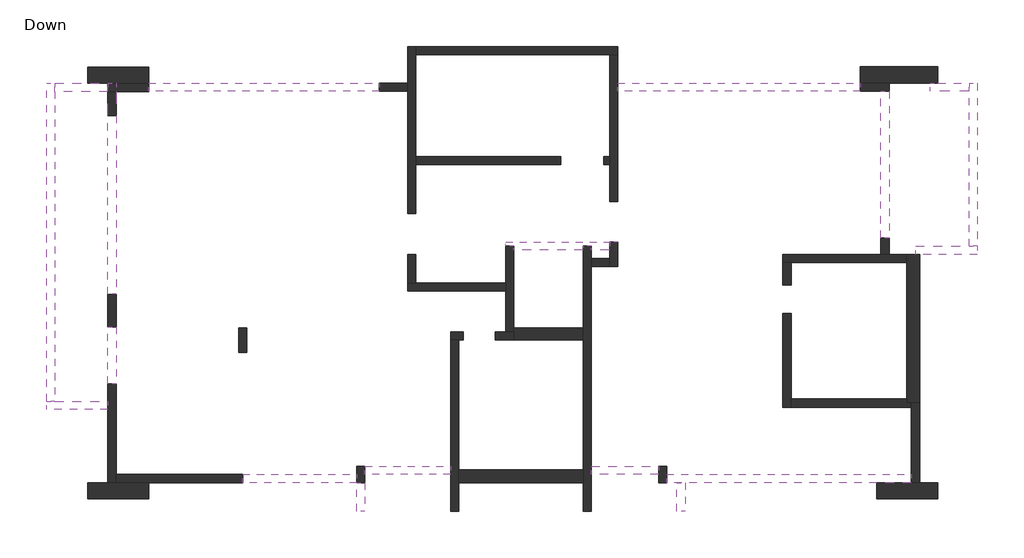
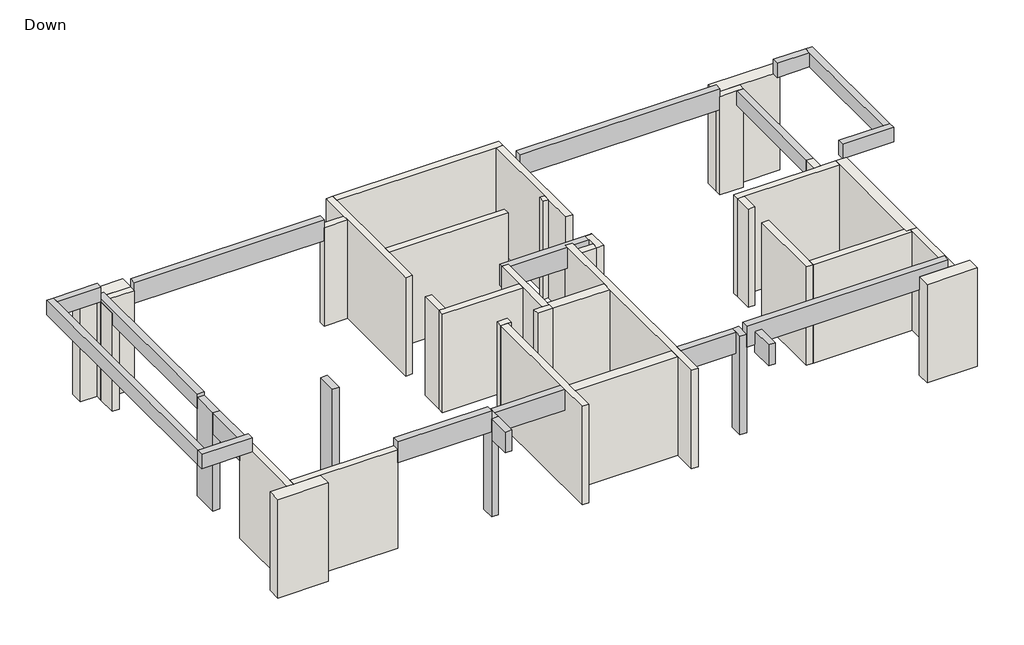
# One storey: 33 walls, 18 beams, 4 columns.
"""IFC4 building model written with IfcOpenShell, lengths in millimetres."""

from ifc_helpers import new_model, si_unit, frame, origin, origin_with_axes, place, context, project, spatial, polyline, outline, extrude, faceted_brep, element, save

model = new_model("IFC4")

# Units and contexts
model_context = context("Model", 3, world=origin())
ifc_project = project(units=[si_unit("LENGTHUNIT", "METRE", prefix="MILLI")], contexts=[model_context])

# Site, building, storey
site = spatial("IfcSite", under=ifc_project)
building = spatial("IfcBuilding", under=site)
storey = spatial("IfcBuildingStorey", under=building, Name="Down", Elevation=0.0)

# Beams
placement = place(None, origin())
element("IfcBeam", 1, ObjectType="Concrete Rectengular Beam : 20/45", at=placement, inside=storey, context=model_context, shape_type="Brep", body=[
    faceted_brep([(-51622.338535, 14321.5649818, 3200.0), (-51822.338535, 14321.5649818, 3200.0), (-51822.338535, 14321.5649818, 2750.0), (-51622.338535, 14321.5649818, 2750.0), (-51622.338535, 19497.0389138, 3200.0), (-51822.338535, 19497.0389138, 3200.0), (-51822.338535, 19497.0389138, 3100.0), (-51822.338535, 19297.0389138, 3100.0), (-51822.338535, 18701.2717181, 3100.0), (-51822.338535, 18701.2717181, 2750.0), (-51622.338535, 18701.2717181, 2750.0), (-51622.338535, 18701.2717181, 3100.0), (-51622.338535, 19297.0389138, 3100.0), (-51622.338535, 19497.0389138, 3100.0)], [[[0, 1, 2, 3]], [[1, 0, 4, 5]], [[2, 1, 5, 6, 7, 8, 9]], [[3, 2, 9, 10]], [[0, 3, 10, 11, 12, 13, 4]], [[5, 4, 13, 6]], [[6, 13, 12, 11, 8, 7]], [[8, 11, 10, 9]]]),
])
element("IfcBeam", 2, ObjectType="Concrete Rectengular Beam : 20/45", at=placement, inside=storey, context=model_context, shape_type="Brep", body=[
    faceted_brep([(-32674.1903869, 19301.2717181, 3100.0), (-32874.1903869, 19301.2717181, 3100.0), (-32874.1903869, 15700.213517, 3100.0), (-32674.1903869, 15700.213517, 3100.0), (-32674.1903869, 19301.2717181, 2650.0), (-32674.1903869, 19301.2717181, 2850.0), (-32674.1903869, 15700.213517, 2650.0), (-32874.1903869, 19301.2717181, 2650.0), (-32874.1903869, 15700.213517, 2650.0), (-32874.1903869, 19301.2717181, 2850.0), (-32874.1903869, 15700.213517, 2850.0)], [[[0, 1, 2, 3]], [[4, 5, 0, 3, 6]], [[7, 4, 6, 8]], [[2, 1, 9, 7, 8, 10]], [[1, 0, 5, 4, 7, 9]], [[3, 2, 10, 8, 6]]]),
])
element("IfcBeam", 3, ObjectType="Concrete Rectengular Beam : 20/45", at=placement, inside=storey, context=model_context, shape_type="Brep", body=[
    faceted_brep([(-32023.9258366, 15500.213517, 3550.0), (-32023.9258366, 15500.213517, 3100.0), (-32023.9258366, 15300.213517, 3100.0), (-32023.9258366, 15300.213517, 3550.0), (-30505.8186523, 15300.213517, 3550.0), (-30505.8186523, 15500.213517, 3550.0), (-30705.8186523, 15500.213517, 3550.0), (-30505.8186523, 15300.213517, 3100.0), (-30705.8186523, 15500.213517, 3100.0), (-30505.8186523, 15500.213517, 3100.0)], [[[0, 1, 2, 3]], [[0, 3, 4, 5, 6]], [[3, 2, 7, 4]], [[2, 1, 8, 9, 7]], [[1, 0, 6, 5, 9, 8]], [[5, 4, 7, 9]]]),
])
element("IfcBeam", 4, ObjectType="Concrete Rectengular Beam : 20/45", at=placement, inside=storey, context=model_context, shape_type="Brep", body=[
    faceted_brep([(-30505.8186523, 19501.2717181, 3550.0), (-30705.8186523, 19501.2717181, 3550.0), (-30705.8186523, 19301.2717181, 3550.0), (-30705.8186523, 15500.213517, 3550.0), (-30505.8186523, 15500.213517, 3550.0), (-30505.8186523, 19501.2717181, 3100.0), (-30505.8186523, 15500.213517, 3100.0), (-30705.8186523, 19501.2717181, 3100.0), (-30705.8186523, 15500.213517, 3100.0), (-30705.8186523, 19301.2717181, 3100.0)], [[[0, 1, 2, 3, 4]], [[5, 0, 4, 6]], [[7, 5, 6, 8, 9]], [[1, 7, 9, 8, 3, 2]], [[1, 0, 5, 7]], [[4, 3, 8, 6]]]),
])
element("IfcBeam", 5, ObjectType="Concrete Rectengular Beam : 20/45", at=placement, inside=storey, context=model_context, shape_type="Brep", body=[
    faceted_brep([(-31665.8186523, 19301.2717181, 3550.0), (-31665.8186523, 19501.2717181, 3550.0), (-31665.8186523, 19501.2717181, 3100.0), (-31665.8186523, 19301.2717181, 3100.0), (-30705.8186523, 19301.2717181, 3550.0), (-30705.8186523, 19501.2717181, 3550.0), (-30705.8186523, 19501.2717181, 3100.0), (-31473.1321858, 19501.2717181, 3100.0), (-30705.8186523, 19301.2717181, 3100.0)], [[[0, 1, 2, 3]], [[1, 0, 4, 5]], [[2, 1, 5, 6, 7]], [[3, 2, 7, 6, 8]], [[0, 3, 8, 4]], [[5, 4, 8, 6]]]),
])
element("IfcBeam", 6, ObjectType="Concrete Rectengular Beam : 20/45", at=placement, inside=storey, context=model_context, shape_type="Brep", body=[
    faceted_brep([(-51822.338535, 11493.9394503, 3550.0), (-51822.338535, 11493.9394503, 3100.0), (-51822.338535, 11693.9394503, 3100.0), (-51822.338535, 11693.9394503, 3550.0), (-53128.1898421, 11693.9394503, 3550.0), (-53328.1898421, 11693.9394503, 3550.0), (-53328.1898421, 11493.9394503, 3550.0), (-53128.1898421, 11693.9394503, 3100.0), (-53328.1898421, 11693.9394503, 3100.0), (-53328.1898421, 11493.9394503, 3100.0)], [[[0, 1, 2, 3]], [[0, 3, 4, 5, 6]], [[3, 2, 7, 8, 5, 4]], [[2, 1, 9, 8, 7]], [[1, 0, 6, 9]], [[6, 5, 8, 9]]]),
])
element("IfcBeam", 7, ObjectType="Concrete Rectengular Beam : 20/45", at=placement, inside=storey, context=model_context, shape_type="Brep", body=[
    faceted_brep([(-53128.1898421, 19497.0389138, 3550.0), (-53328.1898421, 19497.0389138, 3550.0), (-53328.1898421, 11693.9394503, 3550.0), (-53128.1898421, 11693.9394503, 3550.0), (-53128.1898421, 19297.0389138, 3550.0), (-53128.1898421, 19497.0389138, 3100.0), (-53128.1898421, 11693.9394503, 3100.0), (-53128.1898421, 19297.0389138, 3100.0), (-53328.1898421, 19497.0389138, 3100.0), (-53328.1898421, 11693.9394503, 3100.0)], [[[0, 1, 2, 3, 4]], [[5, 0, 4, 3, 6, 7]], [[8, 5, 7, 6, 9]], [[1, 8, 9, 2]], [[3, 2, 9, 6]], [[1, 0, 5, 8]]]),
])
element("IfcBeam", 8, ObjectType="Concrete Rectengular Beam : 20/45", at=placement, inside=storey, context=model_context, shape_type="Brep", body=[
    faceted_brep([(-51822.338535, 19497.0389138, 3550.0), (-51822.338535, 19297.0389138, 3550.0), (-51822.338535, 19297.0389138, 3100.0), (-51822.338535, 19497.0389138, 3100.0), (-51822.338535, 19497.0389138, 3200.0), (-53128.1898421, 19497.0389138, 3550.0), (-53128.1898421, 19297.0389138, 3550.0), (-53128.1898421, 19297.0389138, 3100.0), (-53128.1898421, 19497.0389138, 3100.0)], [[[0, 1, 2, 3, 4]], [[1, 0, 5, 6]], [[2, 1, 6, 7]], [[3, 2, 7, 8]], [[0, 4, 3, 8, 5]], [[6, 5, 8, 7]]]),
])
element("IfcBeam", 9, ObjectType="Concrete Rectengular Beam : 20/66", at=placement, inside=storey, context=model_context, shape_type="SweptSolid", body=[
    extrude(outline(polyline([(-51822.338535, 13521.5649818), (-51622.338535, 13521.5649818), (-51622.338535, 12125.6103424), (-51822.338535, 12125.6103424), (-51822.338535, 13521.5649818)])), frame((0.0, 0.0, 2440.0), z_axis=(0.0, 0.0, 1.0), x_axis=(1.0, 0.0, 0.0)), (0.0, 0.0, 1.0), 660.0),
])
element("IfcBeam", 10, ObjectType="Concrete Rectengular Beam : 20/66", at=placement, inside=storey, context=model_context, shape_type="Brep", body=[
    faceted_brep([(-45722.0604135, 9899.1553159, 3350.0), (-45722.0604135, 9699.1553159, 3350.0), (-45722.0604135, 9699.1553159, 3100.0), (-45722.0604135, 9699.1553159, 2690.0), (-45722.0604135, 9899.1553159, 2690.0), (-45722.0604135, 9899.1553159, 2850.0), (-45722.0604135, 9899.1553159, 3100.0), (-48520.2494744, 9899.1553159, 3350.0), (-48520.2494744, 9899.1553159, 2690.0), (-48520.2494744, 9699.1553159, 2690.0), (-48520.2494744, 9699.1553159, 3350.0)], [[[0, 1, 2, 3, 4, 5, 6]], [[7, 8, 9, 10]], [[1, 0, 7, 10]], [[3, 2, 1, 10, 9]], [[4, 3, 9, 8]], [[0, 6, 5, 4, 8, 7]]]),
])
element("IfcBeam", 11, ObjectType="Concrete Rectengular Beam : 20/66", at=placement, inside=storey, context=model_context, shape_type="Brep", body=[
    faceted_brep([(-45522.0604135, 10099.1553159, 3100.0), (-45522.0604135, 9899.1553159, 3100.0), (-43423.3967361, 9899.1553159, 3100.0), (-43423.3967361, 10099.1553159, 3100.0), (-45522.0604135, 9899.1553159, 2950.0), (-45522.0604135, 9899.1553159, 2440.0), (-43423.3967361, 9899.1553159, 2440.0), (-43423.3967361, 9899.1553159, 2950.0), (-45522.0604135, 10099.1553159, 2440.0), (-43423.3967361, 10099.1553159, 2440.0), (-43423.3967361, 10099.1553159, 2850.0), (-45522.0604135, 10099.1553159, 2850.0)], [[[0, 1, 2, 3]], [[1, 4, 5, 6, 7, 2]], [[5, 8, 9, 6]], [[0, 3, 10, 9, 8, 11]], [[1, 0, 11, 8, 5, 4]], [[3, 2, 7, 6, 9, 10]]]),
])
element("IfcBeam", 12, ObjectType="Concrete Rectengular Beam : 20/66", at=placement, inside=storey, context=model_context, shape_type="Brep", body=[
    faceted_brep([(-38322.0604135, 9899.1553159, 3100.0), (-38322.0604135, 10099.1553159, 3100.0), (-39973.6612863, 10099.1553159, 3100.0), (-39973.6612863, 9899.1553159, 3100.0), (-38322.0604135, 10099.1553159, 2850.0), (-38322.0604135, 10099.1553159, 2440.0), (-39973.6612863, 10099.1553159, 2440.0), (-39973.6612863, 10099.1553159, 2850.0), (-38322.0604135, 9899.1553159, 2440.0), (-39973.6612863, 9899.1553159, 2440.0), (-38322.0604135, 9899.1553159, 2950.0), (-39973.6612863, 9899.1553159, 2950.0)], [[[0, 1, 2, 3]], [[2, 1, 4, 5, 6, 7]], [[5, 8, 9, 6]], [[8, 10, 0, 3, 11, 9]], [[1, 0, 10, 8, 5, 4]], [[3, 2, 7, 6, 9, 11]]]),
])
element("IfcBeam", 13, ObjectType="Concrete Rectengular Beam : 20/66", at=placement, inside=storey, context=model_context, shape_type="Brep", body=[
    faceted_brep([(-32123.9258366, 9899.1553159, 2690.0), (-32123.9258366, 9899.1553159, 2850.0), (-32123.9258366, 9899.1553159, 3100.0), (-32123.9258366, 9899.1553159, 3350.0), (-32123.9258366, 9699.1553159, 3350.0), (-32123.9258366, 9699.1553159, 3100.0), (-32123.9258366, 9700.213517, 3100.0), (-32123.9258366, 9700.213517, 2690.0), (-38123.9258366, 9899.1553159, 3350.0), (-38123.9258366, 9699.1553159, 3350.0), (-38122.0604135, 9899.1553159, 2690.0), (-38122.0604135, 9899.1553159, 2850.0), (-38122.0604135, 9899.1553159, 3100.0), (-38123.9258366, 9899.1553159, 3100.0), (-38122.0604135, 9699.1553159, 2690.0), (-32973.6612863, 9700.213517, 2690.0), (-32973.6612863, 9699.1553159, 2690.0), (-38123.9258366, 9699.1553159, 3100.0), (-38122.0604135, 9699.1553159, 3100.0), (-38122.0604135, 9699.1553159, 2950.0), (-32973.6612863, 9699.1553159, 3100.0), (-32973.6612863, 9700.213517, 3100.0)], [[[0, 1, 2, 3, 4, 5, 6, 7]], [[4, 3, 8, 9]], [[3, 2, 1, 0, 10, 11, 12, 13, 8]], [[14, 10, 0, 7, 15, 16]], [[4, 9, 17, 18, 19, 14, 16, 20, 5]], [[18, 12, 11, 10, 14, 19]], [[12, 18, 17, 13]], [[6, 21, 15, 7]], [[21, 20, 16, 15]], [[20, 21, 6, 5]], [[9, 8, 13, 17]]]),
])
element("IfcBeam", 14, ObjectType="Concrete Rectengular Beam : 20/66", at=placement, inside=storey, context=model_context, shape_type="Brep", body=[
    faceted_brep([(-39322.8676355, 19301.2717181, 3350.0), (-39322.8676355, 19501.2717181, 3350.0), (-39322.8676355, 19501.2717181, 2690.0), (-39322.8676355, 19301.2717181, 2690.0), (-39322.8676355, 19301.2717181, 2850.0), (-39322.8676355, 19301.2717181, 3100.0), (-33373.6612863, 19301.2717181, 3350.0), (-33373.6612863, 19301.2717181, 3100.0), (-33373.6612863, 19301.2717181, 2690.0), (-33373.6612863, 19501.2717181, 2690.0), (-33373.6612863, 19501.2717181, 3100.0), (-33373.6612863, 19501.2717181, 3350.0)], [[[0, 1, 2, 3, 4, 5]], [[6, 7, 8, 9, 10, 11]], [[1, 0, 6, 11]], [[2, 1, 11, 10, 9]], [[3, 2, 9, 8]], [[0, 5, 4, 3, 8, 7, 6]]]),
])
element("IfcBeam", 15, ObjectType="Concrete Rectengular Beam : 20/66", at=placement, inside=storey, context=model_context, shape_type="Brep", body=[
    faceted_brep([(-39322.8676355, 15601.2717181, 3100.0), (-42072.0739847, 15601.2717181, 3100.0), (-42072.0739847, 15501.2717181, 3100.0), (-41872.0739847, 15501.2717181, 3100.0), (-41872.0739847, 15401.2717181, 3100.0), (-40173.6612863, 15401.2717181, 3100.0), (-40173.6612863, 15501.2717181, 3100.0), (-39973.6612863, 15501.2717181, 3100.0), (-39973.6612863, 15401.2717181, 3100.0), (-39522.8676355, 15401.2717181, 3100.0), (-39522.8676355, 15600.7426175, 3100.0), (-39322.8676355, 15600.7426175, 3100.0), (-41872.0739847, 15401.2717181, 2440.0), (-40173.6612863, 15401.2717181, 2440.0), (-42072.0739847, 15601.2717181, 2440.0), (-39322.8676355, 15601.2717181, 2440.0), (-39322.8676355, 15600.7426175, 2440.0), (-39522.8676355, 15600.7426175, 2440.0), (-39522.8676355, 15401.2717181, 2440.0), (-39973.6612863, 15401.2717181, 2440.0), (-39973.6612863, 15501.2717181, 2440.0), (-40173.6612863, 15501.2717181, 2440.0), (-41872.0739847, 15501.2717181, 2440.0), (-42072.0739847, 15501.2717181, 2440.0), (-39322.8676355, 15601.2717181, 2850.0), (-42072.0739847, 15601.2717181, 2850.0), (-39322.8676355, 15600.7426175, 2850.0), (-42072.0739847, 15501.2717181, 2850.0)], [[[0, 1, 2, 3, 4, 5, 6, 7, 8, 9, 10, 11]], [[4, 12, 13, 5]], [[14, 15, 16, 17, 18, 19, 20, 21, 13, 12, 22, 23]], [[1, 0, 24, 15, 14, 25]], [[0, 11, 26, 16, 15, 24]], [[2, 1, 25, 14, 23, 27]], [[17, 10, 9, 18]], [[10, 17, 16, 26, 11]], [[3, 22, 12, 4]], [[22, 3, 2, 27, 23]], [[21, 6, 5, 13]], [[7, 20, 19, 8]], [[6, 21, 20, 7]], [[18, 9, 8, 19]]]),
])
element("IfcBeam", 16, ObjectType="Concrete Rectengular Beam : 20/66", at=placement, inside=storey, context=model_context, shape_type="Brep", body=[
    faceted_brep([(-50823.3967361, 19300.213517, 3350.0), (-50823.3967361, 19500.213517, 3350.0), (-50823.3967361, 19500.213517, 2690.0), (-50823.3967361, 19300.213517, 2690.0), (-50823.3967361, 19300.213517, 2850.0), (-50823.3967361, 19300.213517, 3100.0), (-45172.6030853, 19300.213517, 3350.0), (-45172.6030853, 19300.213517, 3100.0), (-45172.6030853, 19300.213517, 2690.0), (-45172.6030853, 19500.213517, 2690.0), (-45172.6030853, 19500.213517, 3100.0), (-45172.6030853, 19500.213517, 3350.0)], [[[0, 1, 2, 3, 4, 5]], [[6, 7, 8, 9, 10, 11]], [[1, 0, 6, 11]], [[2, 1, 11, 10, 9]], [[3, 2, 9, 8]], [[0, 5, 4, 3, 8, 7, 6]]]),
])
element("IfcBeam", 17, ObjectType="Concrete Rectengular Beam : 20/66", at=placement, inside=storey, context=model_context, shape_type="Brep", body=[
    faceted_brep([(-45522.0604135, 8999.1553159, 3100.0), (-45722.0604135, 8999.1553159, 3100.0), (-45722.0604135, 8999.1553159, 2440.0), (-45522.0604135, 8999.1553159, 2440.0), (-45522.0604135, 8999.6844165, 3100.0), (-45522.0604135, 9699.1553159, 3100.0), (-45722.0604135, 9699.1553159, 3100.0), (-45722.0604135, 9699.1553159, 2440.0), (-45522.0604135, 9699.1553159, 2440.0)], [[[0, 1, 2, 3]], [[1, 0, 4, 5, 6]], [[2, 1, 6, 7]], [[3, 2, 7, 8]], [[0, 3, 8, 5, 4]], [[6, 5, 8, 7]]]),
])
element("IfcBeam", 18, ObjectType="Concrete Rectengular Beam : 20/66", at=placement, inside=storey, context=model_context, shape_type="Brep", body=[
    faceted_brep([(-37673.6612863, 8999.1553159, 3100.0), (-37873.6612863, 8999.1553159, 3100.0), (-37873.6612863, 8999.1553159, 2950.0), (-37873.6612863, 8999.1553159, 2440.0), (-37673.6612863, 8999.1553159, 2440.0), (-37673.6612863, 9699.1553159, 3100.0), (-37673.6612863, 9699.1553159, 2440.0), (-37873.6612863, 9699.1553159, 2440.0), (-37873.6612863, 9699.1553159, 2950.0), (-37873.6612863, 9699.1553159, 3100.0)], [[[0, 1, 2, 3, 4]], [[5, 6, 7, 8, 9]], [[1, 0, 5, 9]], [[3, 2, 1, 9, 8, 7]], [[4, 3, 7, 6]], [[0, 4, 6, 5]]]),
])

# Columns
element("IfcColumn", 19, ObjectType="Concrete Rectengular Column : 20/40", at=placement, inside=storey, context=model_context, shape_type="Brep", body=[
    faceted_brep([(-45522.0604135, 10099.1553159, 0.0), (-45522.0604135, 9699.1553159, 0.0), (-45722.0604135, 9699.1553159, 0.0), (-45722.0604135, 10099.1553159, 0.0), (-45522.0604135, 10099.1553159, 3100.0), (-45522.0604135, 9899.1553159, 3100.0), (-45522.0604135, 9699.1553159, 3100.0), (-45722.0604135, 9699.1553159, 3100.0), (-45722.0604135, 9699.1553159, 2690.0), (-45722.0604135, 9899.1553159, 3100.0), (-45722.0604135, 10099.1553159, 3100.0), (-45722.0604135, 10099.1553159, 2850.0)], [[[0, 1, 2, 3]], [[4, 5, 6, 1, 0]], [[6, 7, 8, 2, 1]], [[7, 9, 10, 11, 3, 2, 8]], [[10, 4, 0, 3, 11]], [[4, 10, 9, 7, 6, 5]]]),
])
element("IfcColumn", 20, ObjectType="Concrete Rectengular Column : 20/40", at=placement, inside=storey, context=model_context, shape_type="Brep", body=[
    faceted_brep([(-38122.0604135, 10099.1553159, 0.0), (-38122.0604135, 9699.1553159, 0.0), (-38322.0604135, 9699.1553159, 0.0), (-38322.0604135, 10099.1553159, 0.0), (-38122.0604135, 10099.1553159, 3100.0), (-38122.0604135, 9899.1553159, 3100.0), (-38122.0604135, 9699.1553159, 3100.0), (-38122.0604135, 10099.1553159, 2850.0), (-38322.0604135, 9699.1553159, 3100.0), (-38322.0604135, 9699.1553159, 2950.0), (-38322.0604135, 9899.1553159, 3100.0), (-38322.0604135, 10099.1553159, 3100.0)], [[[0, 1, 2, 3]], [[4, 5, 6, 1, 0, 7]], [[6, 8, 9, 2, 1]], [[8, 10, 11, 3, 2, 9]], [[11, 4, 7, 0, 3]], [[4, 11, 10, 8, 6, 5]]]),
])
element("IfcColumn", 21, ObjectType="Concrete Rectengular Column : 20/60", at=placement, inside=storey, context=model_context, shape_type="Brep", body=[
    faceted_brep([(-48420.2494744, 13497.0617054, 0.0), (-48420.2494744, 12897.0617054, 0.0), (-48620.2494744, 12897.0617054, 0.0), (-48620.2494744, 13497.0617054, 0.0), (-48420.2494744, 13497.0617054, 3100.0), (-48420.2494744, 12897.0617054, 3100.0), (-48420.2494744, 12897.0617054, 2850.0), (-48420.2494744, 13497.0617054, 2850.0), (-48620.2494744, 12897.0617054, 3100.0), (-48620.2494744, 12897.0617054, 2850.0), (-48620.2494744, 13497.0617054, 3100.0), (-48620.2494744, 13497.0617054, 2850.0)], [[[0, 1, 2, 3]], [[4, 5, 6, 1, 0, 7]], [[5, 8, 9, 2, 1, 6]], [[8, 10, 11, 3, 2, 9]], [[10, 4, 7, 0, 3, 11]], [[4, 10, 8, 5]]]),
])
element("IfcColumn", 22, ObjectType="Concrete Rectengular Column : 20/80", at=placement, inside=storey, context=model_context, shape_type="SweptSolid", body=[
    extrude(outline(polyline([(-51622.338535, 14321.5649818), (-51622.338535, 13521.5649818), (-51822.338535, 13521.5649818), (-51822.338535, 14321.5649818), (-51622.338535, 14321.5649818)])), origin_with_axes(), (0.0, 0.0, 1.0), 3100.0),
])

# Walls
element("IfcWall", 23, ObjectType="20", at=placement, inside=storey, context=model_context, shape_type="Brep", body=[
    faceted_brep([(-50823.3967361, 19497.0389138, 0.0), (-51822.338535, 19497.0389138, 0.0), (-51822.338535, 19497.0389138, 2850.0), (-51822.338535, 19497.0389138, 3100.0), (-50823.3967361, 19497.0389138, 3100.0), (-50823.3967361, 19297.0389138, 0.0), (-50823.3967361, 19297.0389138, 2850.0), (-50823.3967361, 19297.0389138, 3100.0), (-51622.338535, 19297.0389138, 3100.0), (-51822.338535, 19297.0389138, 3100.0), (-51822.338535, 19297.0389138, 0.0), (-51622.338535, 19297.0389138, 0.0), (-50823.3967361, 19300.213517, 3100.0)], [[[0, 1, 2, 3, 4]], [[5, 6, 7, 8, 9, 10, 11]], [[1, 0, 5, 11, 10]], [[4, 3, 9, 8, 7, 12]], [[0, 4, 12, 7, 6, 5]], [[3, 2, 1, 10, 9]]]),
])
element("IfcWall", 24, ObjectType="20", at=placement, inside=storey, context=model_context, shape_type="Brep", body=[
    faceted_brep([(-51822.338535, 19297.0389138, 0.0), (-51822.338535, 18701.2717181, 0.0), (-51822.338535, 18701.2717181, 2750.0), (-51822.338535, 18701.2717181, 3100.0), (-51822.338535, 19297.0389138, 3100.0), (-51622.338535, 19297.0389138, 0.0), (-51622.338535, 19297.0389138, 2850.0), (-51622.338535, 19297.0389138, 3100.0), (-51622.338535, 18701.2717181, 3100.0), (-51622.338535, 18701.2717181, 2750.0), (-51622.338535, 18701.2717181, 0.0)], [[[0, 1, 2, 3, 4]], [[5, 6, 7, 8, 9, 10]], [[1, 0, 5, 10]], [[3, 2, 1, 10, 9, 8]], [[4, 3, 8, 7]], [[0, 4, 7, 6, 5]]]),
])
element("IfcWall", 25, ObjectType="20", at=placement, inside=storey, context=model_context, shape_type="Brep", body=[
    faceted_brep([(-51822.338535, 12125.6103424, 0.0), (-51822.338535, 9699.1553159, 0.0), (-51822.338535, 9699.1553159, 3100.0), (-51822.338535, 11493.9394503, 3100.0), (-51822.338535, 12125.6103424, 3100.0), (-51822.338535, 12125.6103424, 2440.0), (-51622.338535, 12125.6103424, 0.0), (-51622.338535, 12125.6103424, 2440.0), (-51622.338535, 12125.6103424, 3100.0), (-51622.338535, 9899.1553159, 3100.0), (-51622.338535, 9699.1553159, 3100.0), (-51622.338535, 9699.1553159, 0.0), (-51622.338535, 9899.1553159, 0.0)], [[[0, 1, 2, 3, 4, 5]], [[6, 7, 8, 9, 10, 11, 12]], [[1, 0, 6, 12, 11]], [[4, 3, 2, 10, 9, 8]], [[0, 5, 4, 8, 7, 6]], [[2, 1, 11, 10]]]),
])
element("IfcWall", 26, ObjectType="20", at=placement, inside=storey, context=model_context, shape_type="Brep", body=[
    faceted_brep([(-51622.338535, 9699.1553159, 0.0), (-50823.3967361, 9699.1553159, 0.0), (-48522.8676355, 9699.1553159, 0.0), (-48522.8676355, 9699.1553159, 3100.0), (-50823.3967361, 9699.1553159, 3100.0), (-51622.338535, 9699.1553159, 3100.0), (-51622.338535, 9899.1553159, 0.0), (-51622.338535, 9899.1553159, 2850.0), (-51622.338535, 9899.1553159, 3100.0), (-48522.8676355, 9899.1553159, 3100.0), (-48522.8676355, 9899.1553159, 0.0)], [[[0, 1, 2, 3, 4, 5]], [[6, 7, 8, 9, 10]], [[2, 1, 0, 6, 10]], [[3, 2, 10, 9]], [[5, 4, 3, 9, 8]], [[0, 5, 8, 7, 6]]]),
])
element("IfcWall", 27, ObjectType="20", at=placement, inside=storey, context=model_context, shape_type="Brep", body=[
    faceted_brep([(-45172.6030853, 19300.213517, 0.0), (-44472.0739847, 19300.213517, 0.0), (-44472.0739847, 19300.213517, 2850.0), (-44472.0739847, 19300.213517, 3100.0), (-45172.6030853, 19300.213517, 3100.0), (-45172.6030853, 19300.213517, 2690.0), (-45172.6030853, 19500.213517, 0.0), (-45172.6030853, 19500.213517, 2690.0), (-45172.6030853, 19500.213517, 3100.0), (-44472.0739847, 19500.213517, 3100.0), (-44472.0739847, 19500.213517, 0.0)], [[[0, 1, 2, 3, 4, 5]], [[6, 7, 8, 9, 10]], [[1, 0, 6, 10]], [[4, 3, 9, 8]], [[0, 5, 4, 8, 7, 6]], [[3, 2, 1, 10, 9]]]),
])
element("IfcWall", 28, ObjectType="20", at=placement, inside=storey, context=model_context, shape_type="Brep", body=[
    faceted_brep([(-44272.0739847, 16301.2717181, 0.0), (-44272.0739847, 17500.213517, 0.0), (-44272.0739847, 17700.213517, 0.0), (-44272.0739847, 20200.7426175, 0.0), (-44272.0739847, 20400.7426175, 0.0), (-44272.0739847, 20400.7426175, 3100.0), (-44272.0739847, 20200.7426175, 3100.0), (-44272.0739847, 17700.213517, 3100.0), (-44272.0739847, 17500.213517, 3100.0), (-44272.0739847, 16301.2717181, 3100.0), (-44272.0739847, 16301.2717181, 2850.0), (-44472.0739847, 16301.2717181, 0.0), (-44472.0739847, 16301.2717181, 2850.0), (-44472.0739847, 16301.2717181, 3100.0), (-44472.0739847, 19300.213517, 3100.0), (-44472.0739847, 19500.213517, 3100.0), (-44472.0739847, 20400.7426175, 3100.0), (-44472.0739847, 20400.7426175, 0.0), (-44472.0739847, 19500.213517, 0.0), (-44472.0739847, 19300.213517, 0.0)], [[[0, 1, 2, 3, 4, 5, 6, 7, 8, 9, 10]], [[11, 12, 13, 14, 15, 16, 17, 18, 19]], [[4, 3, 2, 1, 0, 11, 19, 18, 17]], [[9, 8, 7, 6, 5, 16, 15, 14, 13]], [[0, 10, 9, 13, 12, 11]], [[5, 4, 17, 16]]]),
])
element("IfcWall", 29, ObjectType="20", at=placement, inside=storey, context=model_context, shape_type="Brep", body=[
    faceted_brep([(-44272.0739847, 20200.7426175, 0.0), (-39522.8676355, 20200.7426175, 0.0), (-39322.8676355, 20200.7426175, 0.0), (-39322.8676355, 20200.7426175, 3100.0), (-39522.8676355, 20200.7426175, 3100.0), (-44272.0739847, 20200.7426175, 3100.0), (-44272.0739847, 20200.7426175, 2850.0), (-44272.0739847, 20400.7426175, 0.0), (-44272.0739847, 20400.7426175, 3100.0), (-39322.8676355, 20400.7426175, 3100.0), (-39322.8676355, 20400.7426175, 0.0)], [[[0, 1, 2, 3, 4, 5, 6]], [[7, 8, 9, 10]], [[2, 1, 0, 7, 10]], [[5, 4, 3, 9, 8]], [[0, 6, 5, 8, 7]], [[3, 2, 10, 9]]]),
])
element("IfcWall", 30, ObjectType="20", at=placement, inside=storey, context=model_context, shape_type="Brep", body=[
    faceted_brep([(-39522.8676355, 20200.7426175, 0.0), (-39522.8676355, 17700.213517, 0.0), (-39522.8676355, 17500.213517, 0.0), (-39522.8676355, 16599.6844165, 0.0), (-39522.8676355, 16599.6844165, 2850.0), (-39522.8676355, 16599.6844165, 3100.0), (-39522.8676355, 17500.213517, 3100.0), (-39522.8676355, 17700.213517, 3100.0), (-39522.8676355, 20200.7426175, 3100.0), (-39522.8676355, 20200.7426175, 2850.0), (-39322.8676355, 20200.7426175, 0.0), (-39322.8676355, 20200.7426175, 3100.0), (-39322.8676355, 19301.2717181, 3100.0), (-39322.8676355, 16599.6844165, 3100.0), (-39322.8676355, 16599.6844165, 2850.0), (-39322.8676355, 16599.6844165, 0.0)], [[[0, 1, 2, 3, 4, 5, 6, 7, 8, 9]], [[10, 11, 12, 13, 14, 15]], [[3, 2, 1, 0, 10, 15]], [[5, 4, 3, 15, 14, 13]], [[8, 7, 6, 5, 13, 12, 11]], [[0, 9, 8, 11, 10]]]),
])
element("IfcWall", 31, ObjectType="20", at=placement, inside=storey, context=model_context, shape_type="Brep", body=[
    faceted_brep([(-39522.8676355, 15600.7426175, 0.0), (-39522.8676355, 15199.6844165, 0.0), (-39522.8676355, 14999.6844165, 0.0), (-39522.8676355, 14999.6844165, 3100.0), (-39522.8676355, 15199.6844165, 3100.0), (-39522.8676355, 15600.7426175, 3100.0), (-39322.8676355, 15600.7426175, 0.0), (-39322.8676355, 15600.7426175, 3100.0), (-39322.8676355, 14999.6844165, 3100.0), (-39322.8676355, 14999.6844165, 2850.0), (-39322.8676355, 14999.6844165, 0.0)], [[[0, 1, 2, 3, 4, 5]], [[6, 7, 8, 9, 10]], [[2, 1, 0, 6, 10]], [[5, 4, 3, 8, 7]], [[0, 5, 7, 6]], [[3, 2, 10, 9, 8]]]),
])
element("IfcWall", 32, ObjectType="20", at=placement, inside=storey, context=model_context, shape_type="Brep", body=[
    faceted_brep([(-39522.8676355, 15199.6844165, 0.0), (-39973.6612863, 15199.6844165, 0.0), (-39973.6612863, 15199.6844165, 3100.0), (-39522.8676355, 15199.6844165, 3100.0), (-39522.8676355, 14999.6844165, 0.0), (-39522.8676355, 14999.6844165, 3100.0), (-39973.6612863, 14999.6844165, 3100.0), (-39973.6612863, 14999.6844165, 2850.0), (-39973.6612863, 14999.6844165, 0.0)], [[[0, 1, 2, 3]], [[4, 5, 6, 7, 8]], [[1, 0, 4, 8]], [[3, 2, 6, 5]], [[0, 3, 5, 4]], [[2, 1, 8, 7, 6]]]),
])
element("IfcWall", 33, ObjectType="20", at=placement, inside=storey, context=model_context, shape_type="Brep", body=[
    faceted_brep([(-40173.6612863, 15501.2717181, 0.0), (-40173.6612863, 13499.6844165, 0.0), (-40173.6612863, 13199.6844165, 0.0), (-40173.6612863, 10009.208226, 0.0), (-40173.6612863, 9699.208226, 0.0), (-40173.6612863, 8999.6844165, 0.0), (-40173.6612863, 8999.6844165, 3100.0), (-40173.6612863, 9699.208226, 3100.0), (-40173.6612863, 10009.208226, 3100.0), (-40173.6612863, 13199.6844165, 3100.0), (-40173.6612863, 13499.6844165, 3100.0), (-40173.6612863, 15401.2717181, 3100.0), (-40173.6612863, 15501.2717181, 3100.0), (-40173.6612863, 15501.2717181, 2440.0), (-39973.6612863, 15501.2717181, 0.0), (-39973.6612863, 15501.2717181, 2440.0), (-39973.6612863, 15501.2717181, 3100.0), (-39973.6612863, 15401.2717181, 3100.0), (-39973.6612863, 15199.6844165, 3100.0), (-39973.6612863, 14999.6844165, 3100.0), (-39973.6612863, 10099.1553159, 3100.0), (-39973.6612863, 9899.1553159, 3100.0), (-39973.6612863, 8999.6844165, 3100.0), (-39973.6612863, 8999.6844165, 0.0), (-39973.6612863, 14999.6844165, 0.0), (-39973.6612863, 15199.6844165, 0.0)], [[[0, 1, 2, 3, 4, 5, 6, 7, 8, 9, 10, 11, 12, 13]], [[14, 15, 16, 17, 18, 19, 20, 21, 22, 23, 24, 25]], [[5, 4, 3, 2, 1, 0, 14, 25, 24, 23]], [[6, 5, 23, 22]], [[12, 11, 10, 9, 8, 7, 6, 22, 21, 20, 19, 18, 17, 16]], [[0, 13, 12, 16, 15, 14]]]),
])
element("IfcWall", 34, ObjectType="20", at=placement, inside=storey, context=model_context, shape_type="Brep", body=[
    faceted_brep([(-43223.3967361, 8999.6844165, 0.0), (-43223.3967361, 9699.208226, 0.0), (-43223.3967361, 10009.208226, 0.0), (-43223.3967361, 13199.6844165, 0.0), (-43223.3967361, 13199.6844165, 2850.0), (-43223.3967361, 13199.6844165, 3100.0), (-43223.3967361, 10009.208226, 3100.0), (-43223.3967361, 9699.208226, 3100.0), (-43223.3967361, 8999.6844165, 3100.0), (-43423.3967361, 8999.6844165, 0.0), (-43423.3967361, 8999.6844165, 2950.0), (-43423.3967361, 8999.6844165, 3100.0), (-43423.3967361, 9899.1553159, 3100.0), (-43423.3967361, 10099.1553159, 3100.0), (-43423.3967361, 13199.6844165, 3100.0), (-43423.3967361, 13199.6844165, 0.0)], [[[0, 1, 2, 3, 4, 5, 6, 7, 8]], [[9, 10, 11, 12, 13, 14, 15]], [[3, 2, 1, 0, 9, 15]], [[8, 7, 6, 5, 14, 13, 12, 11]], [[0, 8, 11, 10, 9]], [[5, 4, 3, 15, 14]]]),
])
element("IfcWall", 35, ObjectType="20", at=placement, inside=storey, context=model_context, shape_type="Brep", body=[
    faceted_brep([(-43423.3967361, 13199.6844165, 0.0), (-43223.3967361, 13199.6844165, 0.0), (-43113.343826, 13199.6844165, 0.0), (-43113.343826, 13199.6844165, 2850.0), (-43113.343826, 13199.6844165, 3100.0), (-43223.3967361, 13199.6844165, 3100.0), (-43423.3967361, 13199.6844165, 3100.0), (-43423.3967361, 13399.6844165, 0.0), (-43423.3967361, 13399.6844165, 2850.0), (-43423.3967361, 13399.6844165, 3100.0), (-43113.343826, 13399.6844165, 3100.0), (-43113.343826, 13399.6844165, 2850.0), (-43113.343826, 13399.6844165, 0.0)], [[[0, 1, 2, 3, 4, 5, 6]], [[7, 8, 9, 10, 11, 12]], [[2, 1, 0, 7, 12]], [[4, 3, 2, 12, 11, 10]], [[6, 5, 4, 10, 9]], [[0, 6, 9, 8, 7]]]),
])
element("IfcWall", 36, ObjectType="20", at=placement, inside=storey, context=model_context, shape_type="Brep", body=[
    faceted_brep([(-42328.1586408, 13199.6844165, 0.0), (-41872.0739847, 13199.6844165, 0.0), (-41872.0739847, 13199.6844165, 3100.0), (-42328.1586408, 13199.6844165, 3100.0), (-42328.1586408, 13199.6844165, 2850.0), (-42328.1586408, 13399.6844165, 0.0), (-42328.1586408, 13399.6844165, 2850.0), (-42328.1586408, 13399.6844165, 3100.0), (-42072.0739847, 13399.6844165, 3100.0), (-41872.0739847, 13399.6844165, 3100.0), (-41872.0739847, 13399.6844165, 0.0), (-42072.0739847, 13399.6844165, 0.0)], [[[0, 1, 2, 3, 4]], [[5, 6, 7, 8, 9, 10, 11]], [[1, 0, 5, 11, 10]], [[3, 2, 9, 8, 7]], [[0, 4, 3, 7, 6, 5]], [[2, 1, 10, 9]]]),
])
element("IfcWall", 37, ObjectType="20", at=placement, inside=storey, context=model_context, shape_type="Brep", body=[
    faceted_brep([(-41872.0739847, 13399.6844165, 0.0), (-41872.0739847, 13499.6844165, 0.0), (-41872.0739847, 15501.2717181, 0.0), (-41872.0739847, 15501.2717181, 3100.0), (-41872.0739847, 13499.6844165, 3100.0), (-41872.0739847, 13399.6844165, 3100.0), (-42072.0739847, 13399.6844165, 0.0), (-42072.0739847, 13399.6844165, 2850.0), (-42072.0739847, 13399.6844165, 3100.0), (-42072.0739847, 14399.6844165, 3100.0), (-42072.0739847, 14599.6844165, 3100.0), (-42072.0739847, 15501.2717181, 3100.0), (-42072.0739847, 15501.2717181, 0.0), (-42072.0739847, 14599.6844165, 0.0), (-42072.0739847, 14399.6844165, 0.0)], [[[0, 1, 2, 3, 4, 5]], [[6, 7, 8, 9, 10, 11, 12, 13, 14]], [[2, 1, 0, 6, 14, 13, 12]], [[3, 2, 12, 11]], [[5, 4, 3, 11, 10, 9, 8]], [[0, 5, 8, 7, 6]]]),
])
element("IfcWall", 38, ObjectType="20", at=placement, inside=storey, context=model_context, shape_type="Brep", body=[
    faceted_brep([(-42072.0739847, 14599.6844165, 0.0), (-44272.0739847, 14599.6844165, 0.0), (-44472.0739847, 14599.6844165, 0.0), (-44472.0739847, 14599.6844165, 3100.0), (-44272.0739847, 14599.6844165, 3100.0), (-42072.0739847, 14599.6844165, 3100.0), (-42072.0739847, 14599.6844165, 2850.0), (-42072.0739847, 14399.6844165, 0.0), (-42072.0739847, 14399.6844165, 2850.0), (-42072.0739847, 14399.6844165, 3100.0), (-44472.0739847, 14399.6844165, 3100.0), (-44472.0739847, 14399.6844165, 2850.0), (-44472.0739847, 14399.6844165, 0.0)], [[[0, 1, 2, 3, 4, 5, 6]], [[7, 8, 9, 10, 11, 12]], [[2, 1, 0, 7, 12]], [[5, 4, 3, 10, 9]], [[0, 6, 5, 9, 8, 7]], [[3, 2, 12, 11, 10]]]),
])
element("IfcWall", 39, ObjectType="20", at=placement, inside=storey, context=model_context, shape_type="Brep", body=[
    faceted_brep([(-44272.0739847, 14599.6844165, 0.0), (-44272.0739847, 15300.213517, 0.0), (-44272.0739847, 15300.213517, 2850.0), (-44272.0739847, 15300.213517, 3100.0), (-44272.0739847, 14599.6844165, 3100.0), (-44272.0739847, 14599.6844165, 2850.0), (-44472.0739847, 14599.6844165, 0.0), (-44472.0739847, 14599.6844165, 3100.0), (-44472.0739847, 15300.213517, 3100.0), (-44472.0739847, 15300.213517, 2850.0), (-44472.0739847, 15300.213517, 0.0)], [[[0, 1, 2, 3, 4, 5]], [[6, 7, 8, 9, 10]], [[1, 0, 6, 10]], [[3, 2, 1, 10, 9, 8]], [[4, 3, 8, 7]], [[0, 5, 4, 7, 6]]]),
])
element("IfcWall", 40, ObjectType="20", at=placement, inside=storey, context=model_context, shape_type="Brep", body=[
    faceted_brep([(-44272.0739847, 17500.213517, 0.0), (-40723.9258366, 17500.213517, 0.0), (-40723.9258366, 17500.213517, 2850.0), (-40723.9258366, 17500.213517, 3100.0), (-44272.0739847, 17500.213517, 3100.0), (-44272.0739847, 17500.213517, 2850.0), (-44272.0739847, 17700.213517, 0.0), (-44272.0739847, 17700.213517, 2850.0), (-44272.0739847, 17700.213517, 3100.0), (-40723.9258366, 17700.213517, 3100.0), (-40723.9258366, 17700.213517, 2850.0), (-40723.9258366, 17700.213517, 0.0)], [[[0, 1, 2, 3, 4, 5]], [[6, 7, 8, 9, 10, 11]], [[1, 0, 6, 11]], [[3, 2, 1, 11, 10, 9]], [[4, 3, 9, 8]], [[0, 5, 4, 8, 7, 6]]]),
])
element("IfcWall", 41, ObjectType="20", at=placement, inside=storey, context=model_context, shape_type="Brep", body=[
    faceted_brep([(-39672.0739847, 17500.213517, 0.0), (-39522.8676355, 17500.213517, 0.0), (-39522.8676355, 17500.213517, 2850.0), (-39522.8676355, 17500.213517, 3100.0), (-39672.0739847, 17500.213517, 3100.0), (-39672.0739847, 17500.213517, 2850.0), (-39672.0739847, 17700.213517, 0.0), (-39672.0739847, 17700.213517, 2850.0), (-39672.0739847, 17700.213517, 3100.0), (-39522.8676355, 17700.213517, 3100.0), (-39522.8676355, 17700.213517, 2850.0), (-39522.8676355, 17700.213517, 0.0)], [[[0, 1, 2, 3, 4, 5]], [[6, 7, 8, 9, 10, 11]], [[1, 0, 6, 11]], [[4, 3, 9, 8]], [[0, 5, 4, 8, 7, 6]], [[3, 2, 1, 11, 10, 9]]]),
])
element("IfcWall", 42, ObjectType="20", at=placement, inside=storey, context=model_context, shape_type="Brep", body=[
    faceted_brep([(-31923.9258366, 9700.213517, 0.0), (-31923.9258366, 11649.9489667, 0.0), (-31923.9258366, 11649.9489667, 3100.0), (-31923.9258366, 9700.213517, 3100.0), (-32123.9258366, 9700.213517, 0.0), (-32123.9258366, 9700.213517, 3100.0), (-32123.9258366, 9899.1553159, 3100.0), (-32123.9258366, 11549.9489667, 3100.0), (-32123.9258366, 11649.9489667, 3100.0), (-32123.9258366, 11649.9489667, 0.0), (-32123.9258366, 11549.9489667, 0.0)], [[[0, 1, 2, 3]], [[4, 5, 6, 7, 8, 9, 10]], [[1, 0, 4, 10, 9]], [[2, 1, 9, 8]], [[3, 2, 8, 7, 6, 5]], [[0, 3, 5, 4]]]),
])
element("IfcWall", 43, ObjectType="20", at=placement, inside=storey, context=model_context, shape_type="Brep", body=[
    faceted_brep([(-32233.9258366, 15300.213517, 0.0), (-32674.1903869, 15300.213517, 0.0), (-32874.1903869, 15300.213517, 0.0), (-35274.1903869, 15300.213517, 0.0), (-35274.1903869, 15300.213517, 2850.0), (-35274.1903869, 15300.213517, 3100.0), (-32874.1903869, 15300.213517, 3100.0), (-32674.1903869, 15300.213517, 3100.0), (-32233.9258366, 15300.213517, 3100.0), (-32233.9258366, 15100.213517, 0.0), (-32233.9258366, 15100.213517, 2850.0), (-32233.9258366, 15100.213517, 3100.0), (-35074.1903869, 15100.213517, 3100.0), (-35274.1903869, 15100.213517, 3100.0), (-35274.1903869, 15100.213517, 0.0), (-35074.1903869, 15100.213517, 0.0)], [[[0, 1, 2, 3, 4, 5, 6, 7, 8]], [[9, 10, 11, 12, 13, 14, 15]], [[3, 2, 1, 0, 9, 15, 14]], [[8, 7, 6, 5, 13, 12, 11]], [[0, 8, 11, 10, 9]], [[5, 4, 3, 14, 13]]]),
])
element("IfcWall", 44, ObjectType="20", at=placement, inside=storey, context=model_context, shape_type="Brep", body=[
    faceted_brep([(-35274.1903869, 15100.213517, 0.0), (-35274.1903869, 14551.0071678, 0.0), (-35274.1903869, 14551.0071678, 2850.0), (-35274.1903869, 14551.0071678, 3100.0), (-35274.1903869, 15100.213517, 3100.0), (-35074.1903869, 15100.213517, 0.0), (-35074.1903869, 15100.213517, 2850.0), (-35074.1903869, 15100.213517, 3100.0), (-35074.1903869, 14551.0071678, 3100.0), (-35074.1903869, 14551.0071678, 2850.0), (-35074.1903869, 14551.0071678, 0.0)], [[[0, 1, 2, 3, 4]], [[5, 6, 7, 8, 9, 10]], [[1, 0, 5, 10]], [[3, 2, 1, 10, 9, 8]], [[4, 3, 8, 7]], [[0, 4, 7, 6, 5]]]),
])
element("IfcWall", 45, ObjectType="20", at=placement, inside=storey, context=model_context, shape_type="Brep", body=[
    faceted_brep([(-35274.1903869, 13846.245263, 0.0), (-35274.1903869, 11549.9489667, 0.0), (-35274.1903869, 11549.9489667, 2850.0), (-35274.1903869, 11549.9489667, 3100.0), (-35274.1903869, 13846.245263, 3100.0), (-35274.1903869, 13846.245263, 2850.0), (-35074.1903869, 13846.245263, 0.0), (-35074.1903869, 13846.245263, 2850.0), (-35074.1903869, 13846.245263, 3100.0), (-35074.1903869, 11749.9489667, 3100.0), (-35074.1903869, 11549.9489667, 3100.0), (-35074.1903869, 11549.9489667, 0.0), (-35074.1903869, 11749.9489667, 0.0)], [[[0, 1, 2, 3, 4, 5]], [[6, 7, 8, 9, 10, 11, 12]], [[1, 0, 6, 12, 11]], [[4, 3, 10, 9, 8]], [[0, 5, 4, 8, 7, 6]], [[3, 2, 1, 11, 10]]]),
])
element("IfcWall", 46, ObjectType="20", at=placement, inside=storey, context=model_context, shape_type="Brep", body=[
    faceted_brep([(-35074.1903869, 11549.9489667, 0.0), (-32123.9258366, 11549.9489667, 0.0), (-32123.9258366, 11549.9489667, 2850.0), (-32123.9258366, 11549.9489667, 3100.0), (-35074.1903869, 11549.9489667, 3100.0), (-35074.1903869, 11749.9489667, 0.0), (-35074.1903869, 11749.9489667, 2850.0), (-35074.1903869, 11749.9489667, 3100.0), (-32233.9258366, 11749.9489667, 3100.0), (-32233.9258366, 11749.9489667, 2850.0), (-32233.9258366, 11749.9489667, 0.0), (-32233.9258366, 11649.9489667, 0.0), (-32123.9258366, 11649.9489667, 0.0), (-32123.9258366, 11649.9489667, 3100.0), (-32233.9258366, 11649.9489667, 3100.0)], [[[0, 1, 2, 3, 4]], [[5, 6, 7, 8, 9, 10]], [[1, 0, 5, 10, 11, 12]], [[4, 3, 13, 14, 8, 7]], [[0, 4, 7, 6, 5]], [[3, 2, 1, 12, 13]], [[12, 11, 14, 13]], [[11, 10, 9, 8, 14]]]),
])
element("IfcWall", 47, ObjectType="20", at=placement, inside=storey, context=model_context, shape_type="Brep", body=[
    faceted_brep([(-32674.1903869, 15300.213517, 0.0), (-32674.1903869, 15700.213517, 0.0), (-32674.1903869, 15700.213517, 2650.0), (-32674.1903869, 15700.213517, 3100.0), (-32674.1903869, 15300.213517, 3100.0), (-32674.1903869, 15300.213517, 2850.0), (-32874.1903869, 15300.213517, 0.0), (-32874.1903869, 15300.213517, 2850.0), (-32874.1903869, 15300.213517, 3100.0), (-32874.1903869, 15700.213517, 3100.0), (-32874.1903869, 15700.213517, 2650.0), (-32874.1903869, 15700.213517, 0.0)], [[[0, 1, 2, 3, 4, 5]], [[6, 7, 8, 9, 10, 11]], [[1, 0, 6, 11]], [[3, 2, 1, 11, 10, 9]], [[4, 3, 9, 8]], [[0, 5, 4, 8, 7, 6]]]),
])
element("IfcWall", 48, ObjectType="20", at=placement, inside=storey, context=model_context, shape_type="Brep", body=[
    faceted_brep([(-33373.6612863, 19301.2717181, 0.0), (-32673.1321858, 19301.2717181, 0.0), (-32673.1321858, 19301.2717181, 2850.0), (-32673.1321858, 19301.2717181, 3100.0), (-32674.1903869, 19301.2717181, 3100.0), (-32874.1903869, 19301.2717181, 3100.0), (-33373.6612863, 19301.2717181, 3100.0), (-33373.6612863, 19301.2717181, 2690.0), (-33373.6612863, 19501.2717181, 0.0), (-33373.6612863, 19501.2717181, 2690.0), (-33373.6612863, 19501.2717181, 3100.0), (-32673.1321858, 19501.2717181, 3100.0), (-32673.1321858, 19501.2717181, 2850.0), (-32673.1321858, 19501.2717181, 0.0)], [[[0, 1, 2, 3, 4, 5, 6, 7]], [[8, 9, 10, 11, 12, 13]], [[1, 0, 8, 13]], [[3, 2, 1, 13, 12, 11]], [[6, 5, 4, 3, 11, 10]], [[0, 7, 6, 10, 9, 8]]]),
])
element("IfcWall", 49, ObjectType="30", at=placement, inside=storey, context=model_context, shape_type="Brep", body=[
    faceted_brep([(-41872.0739847, 13199.6844165, 0.0), (-40173.6612863, 13199.6844165, 0.0), (-40173.6612863, 13199.6844165, 2850.0), (-40173.6612863, 13199.6844165, 3100.0), (-41872.0739847, 13199.6844165, 3100.0), (-41872.0739847, 13499.6844165, 0.0), (-41872.0739847, 13499.6844165, 3100.0), (-40173.6612863, 13499.6844165, 3100.0), (-40173.6612863, 13499.6844165, 0.0), (-41872.0739847, 13399.6844165, 0.0), (-41872.0739847, 13399.6844165, 3100.0)], [[[0, 1, 2, 3, 4]], [[5, 6, 7, 8]], [[1, 0, 9, 5, 8]], [[4, 3, 7, 6, 10]], [[0, 4, 10, 6, 5, 9]], [[3, 2, 1, 8, 7]]]),
])
element("IfcWall", 50, ObjectType="31", at=placement, inside=storey, context=model_context, shape_type="Brep", body=[
    faceted_brep([(-40173.6612863, 10009.208226, 0.0), (-43223.3967361, 10009.208226, 0.0), (-43223.3967361, 10009.208226, 2850.0), (-43223.3967361, 10009.208226, 3100.0), (-40173.6612863, 10009.208226, 3100.0), (-40173.6612863, 10009.208226, 2850.0), (-40173.6612863, 9699.208226, 0.0), (-40173.6612863, 9699.208226, 3100.0), (-43223.3967361, 9699.208226, 3100.0), (-43223.3967361, 9699.208226, 0.0)], [[[0, 1, 2, 3, 4, 5]], [[6, 7, 8, 9]], [[1, 0, 6, 9]], [[4, 3, 8, 7]], [[3, 2, 1, 9, 8]], [[0, 5, 4, 7, 6]]]),
])
element("IfcWall", 51, ObjectType="31", at=placement, inside=storey, context=model_context, shape_type="Brep", body=[
    faceted_brep([(-31923.9258366, 11649.9489667, 0.0), (-31923.9258366, 15300.213517, 0.0), (-31923.9258366, 15300.213517, 3100.0), (-31923.9258366, 11649.9489667, 3100.0), (-32233.9258366, 11649.9489667, 0.0), (-32233.9258366, 11649.9489667, 3100.0), (-32233.9258366, 11749.9489667, 3100.0), (-32233.9258366, 15100.213517, 3100.0), (-32233.9258366, 15300.213517, 3100.0), (-32233.9258366, 15300.213517, 0.0), (-32233.9258366, 15100.213517, 0.0), (-32233.9258366, 11749.9489667, 0.0), (-32123.9258366, 11649.9489667, 0.0), (-32123.9258366, 11649.9489667, 3100.0)], [[[0, 1, 2, 3]], [[4, 5, 6, 7, 8, 9, 10, 11]], [[1, 0, 12, 4, 11, 10, 9]], [[3, 2, 8, 7, 6, 5, 13]], [[0, 3, 13, 5, 4, 12]], [[2, 1, 9, 8]]]),
])
element("IfcWall", 52, ObjectType="40", at=placement, inside=storey, context=model_context, shape_type="Brep", body=[
    faceted_brep([(-52321.8094345, 19497.0389138, 0.0), (-51822.338535, 19497.0389138, 0.0), (-50823.3967361, 19497.0389138, 0.0), (-50823.3967361, 19497.0389138, 3100.0), (-51822.338535, 19497.0389138, 3100.0), (-52321.8094345, 19497.0389138, 3100.0), (-52321.8094345, 19897.0389138, 0.0), (-52321.8094345, 19897.0389138, 3100.0), (-50823.3967361, 19897.0389138, 3100.0), (-50823.3967361, 19897.0389138, 0.0)], [[[0, 1, 2, 3, 4, 5]], [[6, 7, 8, 9]], [[2, 1, 0, 6, 9]], [[3, 2, 9, 8]], [[5, 4, 3, 8, 7]], [[0, 5, 7, 6]]]),
])
element("IfcWall", 53, ObjectType="40", at=placement, inside=storey, context=model_context, shape_type="Brep", body=[
    faceted_brep([(-52321.8094345, 9299.1553159, 0.0), (-50823.3967361, 9299.1553159, 0.0), (-50823.3967361, 9299.1553159, 3100.0), (-52321.8094345, 9299.1553159, 3100.0), (-52321.8094345, 9699.1553159, 0.0), (-52321.8094345, 9699.1553159, 3100.0), (-51822.338535, 9699.1553159, 3100.0), (-51622.338535, 9699.1553159, 3100.0), (-50823.3967361, 9699.1553159, 3100.0), (-50823.3967361, 9699.1553159, 0.0), (-51622.338535, 9699.1553159, 0.0), (-51822.338535, 9699.1553159, 0.0)], [[[0, 1, 2, 3]], [[4, 5, 6, 7, 8, 9, 10, 11]], [[1, 0, 4, 11, 10, 9]], [[2, 1, 9, 8]], [[3, 2, 8, 7, 6, 5]], [[0, 3, 5, 4]]]),
])
element("IfcWall", 54, ObjectType="40", at=placement, inside=storey, context=model_context, shape_type="Brep", body=[
    faceted_brep([(-31473.1321858, 9700.213517, 0.0), (-31923.9258366, 9700.213517, 0.0), (-32123.9258366, 9700.213517, 0.0), (-32973.6612863, 9700.213517, 0.0), (-32973.6612863, 9700.213517, 2690.0), (-32973.6612863, 9700.213517, 3100.0), (-32123.9258366, 9700.213517, 3100.0), (-31923.9258366, 9700.213517, 3100.0), (-31473.1321858, 9700.213517, 3100.0), (-31473.1321858, 9300.213517, 0.0), (-31473.1321858, 9300.213517, 3100.0), (-32973.6612863, 9300.213517, 3100.0), (-32973.6612863, 9300.213517, 0.0), (-32973.6612863, 9699.1553159, 3100.0)], [[[0, 1, 2, 3, 4, 5, 6, 7, 8]], [[9, 10, 11, 12]], [[3, 2, 1, 0, 9, 12]], [[5, 4, 3, 12, 11, 13]], [[8, 7, 6, 5, 13, 11, 10]], [[0, 8, 10, 9]]]),
])
element("IfcWall", 55, ObjectType="40", at=placement, inside=storey, context=model_context, shape_type="Brep", body=[
    faceted_brep([(-31473.1321858, 19901.2717181, 0.0), (-33373.6612863, 19901.2717181, 0.0), (-33373.6612863, 19901.2717181, 3100.0), (-31473.1321858, 19901.2717181, 3100.0), (-31473.1321858, 19501.2717181, 0.0), (-31473.1321858, 19501.2717181, 2850.0), (-31473.1321858, 19501.2717181, 3100.0), (-32673.1321858, 19501.2717181, 3100.0), (-33373.6612863, 19501.2717181, 3100.0), (-33373.6612863, 19501.2717181, 0.0), (-32673.1321858, 19501.2717181, 0.0), (-31473.1321858, 19506.2717181, 3100.0)], [[[0, 1, 2, 3]], [[4, 5, 6, 7, 8, 9, 10]], [[1, 0, 4, 10, 9]], [[2, 1, 9, 8]], [[3, 2, 8, 7, 6, 11]], [[0, 3, 11, 6, 5, 4]]]),
])

save(model, "model.ifc")

# Revit data of these elements
# Project information
#   Project Issue Date = "Issue Date"
#   Project Status = "Project Status"
#   Client Name = "לקוח"
#   Project Address = "Enter address here"
#   Project Name = "Project 042"
#   Project Number = "מספר פרויקט"
# Type "Concrete Rectengular Beam : 20/45"
#   Length [instance default] = 152.4 cm
#   b = 20 cm
#   h = 45 cm
#   Structural Material [instance default] = Concrete
#   Assembly Code = ""
# Type "Concrete Rectengular Beam : 20/66"
#   Length [instance default] = 152.4 cm
#   b = 20 cm
#   h = 66 cm
#   Structural Material [instance default] = Concrete
#   Assembly Code = ""
# Type "Concrete Rectengular Column : 20/40"
#   b = 20 cm
#   h = 40 cm
#   Structural Material [instance default] = Concrete
# Type "Concrete Rectengular Column : 20/60"
#   b = 20 cm
#   h = 60 cm
#   Structural Material [instance default] = Concrete
# Type "Concrete Rectengular Column : 20/80"
#   b = 20 cm
#   h = 80 cm
#   Structural Material [instance default] = Concrete
# Type "20"
#   Layers, outside or top first: 20 cm "Concrete" (function 1)
# Type "30"
#   Layers, outside or top first: 30 cm "Concrete" (function 1)
# Type "31"
#   Layers, outside or top first: 31 cm "Concrete" (function 1)
# Type "40"
#   Layers, outside or top first: 40 cm "Concrete" (function 1)
# Element 1 (IfcBeam, "Concrete Rectengular Beam : 20/45")
#   Comments = ""
#   Mark = "B1"
#   SOFiSTiK_AMG_Comments = ""
#   SOFiSTiK_AMG_Scheduled = yes
#   SOFiSTiK_AMG_Adjusted = yes
#   Structural Material = Concrete
#   Phase Created = New Construction
#   Materials on its faces: "Concrete"
# Element 2 (IfcBeam, "Concrete Rectengular Beam : 20/45")
#   Comments = ""
#   Mark = "B2"
#   SOFiSTiK_AMG_Comments = ""
#   SOFiSTiK_AMG_Scheduled = yes
#   SOFiSTiK_AMG_Adjusted = yes
#   Structural Material = Concrete
#   Phase Created = New Construction
#   Materials on its faces: "Concrete"
# Element 3 (IfcBeam, "Concrete Rectengular Beam : 20/45")
#   Comments = ""
#   Mark = "B3"
#   SOFiSTiK_AMG_Comments = ""
#   SOFiSTiK_AMG_Scheduled = yes
#   SOFiSTiK_AMG_Adjusted = yes
#   Structural Material = Concrete
#   Phase Created = New Construction
#   Materials on its faces: "Concrete"
# Element 4 (IfcBeam, "Concrete Rectengular Beam : 20/45")
#   Comments = ""
#   Mark = "B4"
#   SOFiSTiK_AMG_Comments = ""
#   SOFiSTiK_AMG_Scheduled = yes
#   SOFiSTiK_AMG_Adjusted = yes
#   Structural Material = Concrete
#   Phase Created = New Construction
#   Materials on its faces: "Concrete"
# Element 5 (IfcBeam, "Concrete Rectengular Beam : 20/45")
#   Comments = ""
#   Mark = "B5"
#   SOFiSTiK_AMG_Comments = ""
#   SOFiSTiK_AMG_Scheduled = yes
#   SOFiSTiK_AMG_Adjusted = yes
#   Structural Material = Concrete
#   Phase Created = New Construction
#   Materials on its faces: "Concrete"
# Element 6 (IfcBeam, "Concrete Rectengular Beam : 20/45")
#   Comments = ""
#   Mark = "B6"
#   SOFiSTiK_AMG_Comments = ""
#   SOFiSTiK_AMG_Scheduled = yes
#   SOFiSTiK_AMG_Adjusted = yes
#   Structural Material = Concrete
#   Phase Created = New Construction
#   Materials on its faces: "Concrete"
# Element 7 (IfcBeam, "Concrete Rectengular Beam : 20/45")
#   Comments = ""
#   Mark = "B7"
#   SOFiSTiK_AMG_Comments = ""
#   SOFiSTiK_AMG_Scheduled = yes
#   SOFiSTiK_AMG_Adjusted = yes
#   Structural Material = Concrete
#   Phase Created = New Construction
#   Materials on its faces: "Concrete"
# Element 8 (IfcBeam, "Concrete Rectengular Beam : 20/45")
#   Comments = ""
#   Mark = "B8"
#   SOFiSTiK_AMG_Comments = ""
#   SOFiSTiK_AMG_Scheduled = yes
#   SOFiSTiK_AMG_Adjusted = yes
#   Structural Material = Concrete
#   Phase Created = New Construction
#   Materials on its faces: "Concrete"
# Element 9 (IfcBeam, "Concrete Rectengular Beam : 20/66")
#   Comments = ""
#   Mark = "B9"
#   SOFiSTiK_AMG_Comments = ""
#   SOFiSTiK_AMG_Scheduled = yes
#   SOFiSTiK_AMG_Adjusted = yes
#   Structural Material = Concrete
#   Phase Created = New Construction
#   Materials on its faces: "Concrete"
# Element 10 (IfcBeam, "Concrete Rectengular Beam : 20/66")
#   Comments = ""
#   Mark = "B10"
#   SOFiSTiK_AMG_Comments = ""
#   SOFiSTiK_AMG_Scheduled = yes
#   SOFiSTiK_AMG_Adjusted = yes
#   Structural Material = Concrete
#   Phase Created = New Construction
#   Materials on its faces: "Concrete"
# Element 11 (IfcBeam, "Concrete Rectengular Beam : 20/66")
#   Comments = ""
#   Mark = "B11"
#   SOFiSTiK_AMG_Comments = ""
#   SOFiSTiK_AMG_Scheduled = yes
#   SOFiSTiK_AMG_Adjusted = yes
#   Structural Material = Concrete
#   Phase Created = New Construction
#   Materials on its faces: "Concrete"
# Element 12 (IfcBeam, "Concrete Rectengular Beam : 20/66")
#   Comments = ""
#   Mark = "B12"
#   SOFiSTiK_AMG_Comments = ""
#   SOFiSTiK_AMG_Scheduled = yes
#   SOFiSTiK_AMG_Adjusted = yes
#   Structural Material = Concrete
#   Phase Created = New Construction
#   Materials on its faces: "Concrete"
# Element 13 (IfcBeam, "Concrete Rectengular Beam : 20/66")
#   Comments = ""
#   Mark = "B13"
#   SOFiSTiK_AMG_Comments = ""
#   SOFiSTiK_AMG_Scheduled = yes
#   SOFiSTiK_AMG_Adjusted = yes
#   Structural Material = Concrete
#   Phase Created = New Construction
#   Materials on its faces: "Concrete"
# Element 14 (IfcBeam, "Concrete Rectengular Beam : 20/66")
#   Comments = ""
#   Mark = "B14"
#   SOFiSTiK_AMG_Comments = ""
#   SOFiSTiK_AMG_Scheduled = yes
#   SOFiSTiK_AMG_Adjusted = yes
#   Structural Material = Concrete
#   Phase Created = New Construction
#   Materials on its faces: "Concrete"
# Element 15 (IfcBeam, "Concrete Rectengular Beam : 20/66")
#   Comments = ""
#   Mark = "B15"
#   SOFiSTiK_AMG_Comments = ""
#   SOFiSTiK_AMG_Scheduled = yes
#   SOFiSTiK_AMG_Adjusted = yes
#   Structural Material = Concrete
#   Phase Created = New Construction
#   Materials on its faces: "Concrete"
# Element 16 (IfcBeam, "Concrete Rectengular Beam : 20/66")
#   Comments = ""
#   Mark = "B16"
#   SOFiSTiK_AMG_Comments = ""
#   SOFiSTiK_AMG_Scheduled = yes
#   SOFiSTiK_AMG_Adjusted = yes
#   Structural Material = Concrete
#   Phase Created = New Construction
#   Materials on its faces: "Concrete"
# Element 17 (IfcBeam, "Concrete Rectengular Beam : 20/66")
#   Comments = ""
#   Mark = "B17"
#   SOFiSTiK_AMG_Comments = ""
#   SOFiSTiK_AMG_Scheduled = yes
#   SOFiSTiK_AMG_Adjusted = yes
#   Structural Material = Concrete
#   Phase Created = New Construction
#   Materials on its faces: "Concrete"
# Element 18 (IfcBeam, "Concrete Rectengular Beam : 20/66")
#   Comments = ""
#   Mark = "B18"
#   SOFiSTiK_AMG_Comments = ""
#   SOFiSTiK_AMG_Scheduled = yes
#   SOFiSTiK_AMG_Adjusted = yes
#   Structural Material = Concrete
#   Phase Created = New Construction
#   Materials on its faces: "Concrete"
# Element 19 (IfcColumn, "Concrete Rectengular Column : 20/40")
#   Comments = ""
#   Mark = "C1"
#   SOFiSTiK_AMG_Comments = ""
#   SOFiSTiK_AMG_Scheduled = yes
#   SOFiSTiK_AMG_Adjusted = yes
#   Structural Material = Concrete
#   Phase Created = New Construction
#   Materials on its faces: "Concrete"
# Element 20 (IfcColumn, "Concrete Rectengular Column : 20/40")
#   Comments = ""
#   Mark = "C2"
#   SOFiSTiK_AMG_Comments = ""
#   SOFiSTiK_AMG_Scheduled = yes
#   SOFiSTiK_AMG_Adjusted = yes
#   Structural Material = Concrete
#   Phase Created = New Construction
#   Materials on its faces: "Concrete"
# Element 21 (IfcColumn, "Concrete Rectengular Column : 20/60")
#   Comments = ""
#   Mark = "C3"
#   SOFiSTiK_AMG_Comments = ""
#   SOFiSTiK_AMG_Scheduled = yes
#   SOFiSTiK_AMG_Adjusted = yes
#   Structural Material = Concrete
#   Phase Created = New Construction
#   Materials on its faces: "Concrete"
# Element 22 (IfcColumn, "Concrete Rectengular Column : 20/80")
#   Comments = ""
#   Mark = "C4"
#   SOFiSTiK_AMG_Comments = ""
#   SOFiSTiK_AMG_Scheduled = yes
#   SOFiSTiK_AMG_Adjusted = yes
#   Structural Material = Concrete
#   Phase Created = New Construction
#   Materials on its faces: "Concrete"
# Element 23 (IfcWall, "20")
#   Comments = ""
#   Mark = "W5"
#   SOFiSTiK_EdgeZones = "W5"
